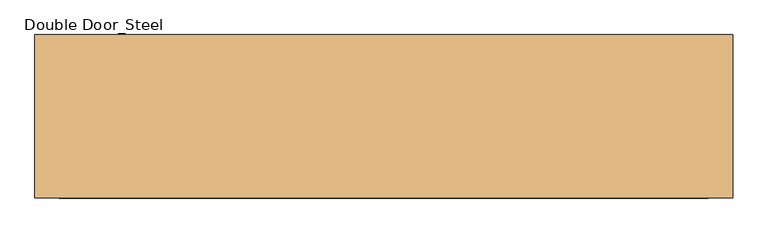
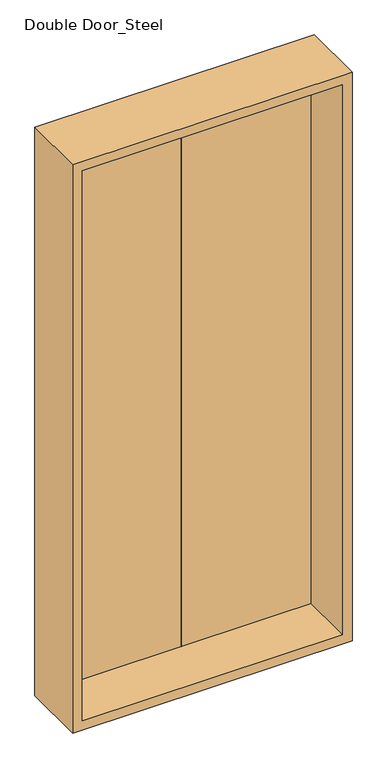
"""IFC4 building model written with IfcOpenShell, lengths in millimetres: door geometry, Double Door_Steel : H_DR_AMB_Double Door_Steel_W1000xH2150."""

from ifc_helpers import new_model, si_unit, frame, origin, place, context, project, spatial, polyline, outline, extrude, faceted_brep, source, transform, mapped, element, save


def double_door_steel_898613e4(model_context):
    return source(origin(), model_context, "Body", "SolidModel", [
        extrude(outline(polyline([(480.0, 77.0), (0.0, 77.0), (0.0, 117.0), (480.0, 117.0), (480.0, 77.0)])), frame((0.0, 0.0, 20.0), z_axis=(0.0, 0.0, 1.0), x_axis=(1.0, 0.0, 0.0)), (0.0, 0.0, 1.0), 2110.0),
        extrude(outline(polyline([(0.0, 77.0), (-480.0, 77.0), (-480.0, 117.0), (0.0, 117.0), (0.0, 77.0)])), frame((0.0, 0.0, 20.0), z_axis=(0.0, 0.0, 1.0), x_axis=(1.0, 0.0, 0.0)), (0.0, 0.0, 1.0), 2110.0),
        faceted_brep([(500.0, -117.0, 0.0), (500.0, 117.0, 0.0), (500.0, 117.0, 2150.0), (500.0, -117.0, 2150.0), (-500.0, 117.0, 2150.0), (-500.0, -117.0, 2150.0), (-500.0, 117.0, 0.0), (480.0, 117.0, 2130.0), (-480.0, 117.0, 2130.0), (-480.0, 117.0, 20.0), (480.0, 117.0, 20.0), (-500.0, -117.0, 0.0), (465.0, -117.0, 35.0), (-465.0, -117.0, 35.0), (-465.0, -117.0, 2115.0), (465.0, -117.0, 2115.0), (465.0, 77.0, 35.0), (465.0, 77.0, 2115.0), (-465.0, 77.0, 2115.0), (-465.0, 77.0, 35.0), (480.0, 77.0, 20.0), (-480.0, 77.0, 20.0), (-480.0, 77.0, 2130.0), (480.0, 77.0, 2130.0)], [[[0, 1, 2, 3]], [[3, 2, 4, 5]], [[1, 6, 4, 2], [7, 8, 9, 10]], [[5, 4, 6, 11]], [[3, 5, 11, 0], [12, 13, 14, 15]], [[16, 12, 15, 17]], [[17, 15, 14, 18]], [[18, 14, 13, 19]], [[20, 21, 22, 23], [17, 18, 19, 16]], [[10, 20, 23, 7]], [[7, 23, 22, 8]], [[8, 22, 21, 9]], [[11, 6, 1, 0]], [[19, 13, 12, 16]], [[9, 21, 20, 10]]]),
    ])


if __name__ == "__main__":
    model = new_model("IFC4")
    model_context = context("Model", 3, world=origin())
    ifc_project = project(units=[si_unit("LENGTHUNIT", "METRE", prefix="MILLI")], contexts=[model_context])
    site = spatial("IfcSite", under=ifc_project)
    building = spatial("IfcBuilding", under=site)
    placement = place(None, origin())
    double_door_steel_shape = double_door_steel_898613e4(model_context)
    element("IfcDoor", 1, ObjectType="Double Door_Steel : H_DR_AMB_Double Door_Steel_W1000xH2150", at=placement, inside=building, context=model_context, shape_type="MappedRepresentation", body=[
        mapped(double_door_steel_shape, transform((0.0, 0.0, 0.0), x_axis=(1.0, 0.0, 0.0), y_axis=(0.0, 1.0, 0.0), z_axis=(0.0, 0.0, 1.0))),
    ])
    save(model, "model.ifc")

# Revit data of these elements
# Type "Double Door_Steel : H_DR_AMB_Double Door_Steel_W1000xH2150"
#   Type Mark = "366"
#   프레임 = ""
#   철물 = ""
#   유리/마감 = ""
#   위치/개소 = ""
#   부호 = "1/SD"
#   문번호 = ""
#   문기호 = "SD"
#   Analytic Construction = "<None>"
#   Height = 2150.000 mm
#   Width = 1000.000 mm
#   Define Thermal Properties by = 1
#   문 틀 = none
#   문 = none
#   Function = (empty or 0)
#   Assembly Code = ""
#   Wall Closure = (empty or 0)
